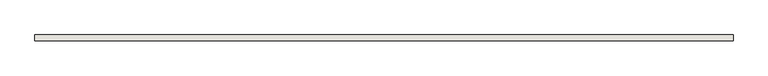
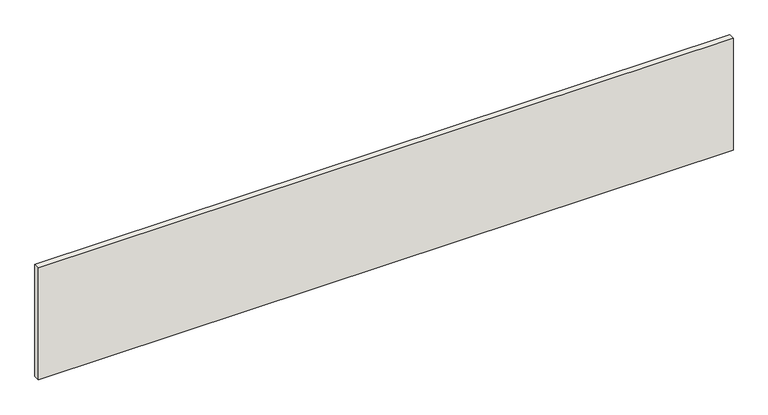
"""IFC4 building model written with IfcOpenShell, lengths in millimetres: wall geometry, 0_3d."""

from ifc_helpers import new_model, si_unit, origin, origin_with_axes, place, context, project, spatial, polyline, outline, extrude, source, transform, mapped, element, save


def wall_6ccf209a(model_context):
    return source(origin(), model_context, "Body", "SweptSolid", [
        extrude(outline(polyline([(5870.0, 50.0), (5870.0, 0.0), (0.0, 0.0), (0.0, 50.0), (5870.0, 50.0)])), origin_with_axes(), (0.0, 0.0, 1.0), 1000.0),
    ])


if __name__ == "__main__":
    model = new_model("IFC4")
    model_context = context("Model", 3, world=origin())
    ifc_project = project(units=[si_unit("LENGTHUNIT", "METRE", prefix="MILLI")], contexts=[model_context])
    site = spatial("IfcSite", under=ifc_project)
    building = spatial("IfcBuilding", under=site)
    placement = place(None, origin())
    wall_shape = wall_6ccf209a(model_context)
    element("IfcWall", 1, ObjectType="0_3d", at=placement, inside=building, context=model_context, shape_type="MappedRepresentation", body=[
        mapped(wall_shape, transform((0.0, 0.0, 0.0), x_axis=(1.0, 0.0, 0.0), y_axis=(0.0, 1.0, 0.0), z_axis=(0.0, 0.0, 1.0))),
    ])
    save(model, "model.ifc")

# Revit data of these elements
# Element 1 (IfcWall, "0_3d")
#   Materials on its faces: "material wardrobe b 1"
# Materials
#   "material wardrobe b 1": class "Unassigned", colour RGB 128 128 128, transparency 0
